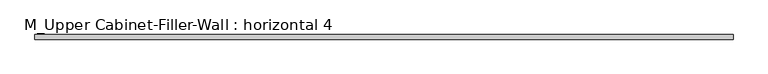
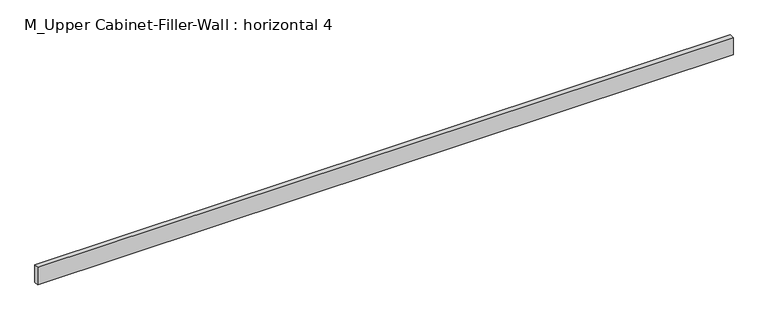
"""IFC4 building model written with IfcOpenShell, lengths in millimetres: furniture geometry, M_Upper Cabinet-Filler-Wall : horizontal 4."""

from ifc_helpers import new_model, si_unit, frame, origin, place, context, project, spatial, polyline, outline, extrude, source, transform, mapped, element, save


def m_upper_cabinet_filler_wall_horizontal_4_0c22a44f(model_context):
    return source(origin(), model_context, "Body", "SweptSolid", [
        extrude(outline(polyline([(-1411.6788372, 38.1), (-1411.6788372, 57.15), (1471.2211628, 57.15), (1471.2211628, 38.1), (-1411.6788372, 38.1)])), frame((0.0, 0.0, 1923.8), z_axis=(0.0, 0.0, 1.0), x_axis=(1.0, 0.0, 0.0)), (0.0, 0.0, 1.0), 76.2),
    ])


if __name__ == "__main__":
    model = new_model("IFC4")
    model_context = context("Model", 3, world=origin())
    ifc_project = project(units=[si_unit("LENGTHUNIT", "METRE", prefix="MILLI")], contexts=[model_context])
    site = spatial("IfcSite", under=ifc_project)
    building = spatial("IfcBuilding", under=site)
    placement = place(None, origin())
    m_upper_cabinet_filler_wall_horizontal_4_shape = m_upper_cabinet_filler_wall_horizontal_4_0c22a44f(model_context)
    element("IfcFurniture", 1, ObjectType="M_Upper Cabinet-Filler-Wall : horizontal 4", at=placement, inside=building, context=model_context, shape_type="MappedRepresentation", body=[
        mapped(m_upper_cabinet_filler_wall_horizontal_4_shape, transform((0.0, 0.0, 0.0), x_axis=(1.0, 0.0, 0.0), y_axis=(0.0, 1.0, 0.0), z_axis=(0.0, 0.0, 1.0))),
    ])
    save(model, "model.ifc")

# Revit data of these elements
# Type "M_Upper Cabinet-Filler-Wall : horizontal 4"
#   Depth = 0' - 1"
#   Height = 0' - 3"
#   Top Of Cabinet = 6' - 6.74016"
#   Width = 9' - 5 1/2"
#   Cabinet Material = none
#   Default Elevation = 0
# Element 1 (IfcFurniture, "M_Upper Cabinet-Filler-Wall : horizontal 4")
#   Materials on its faces: "Cabinets"
# Materials
#   "Cabinets": class "Miscellaneous", colour RGB 249 249 249, transparency 0
